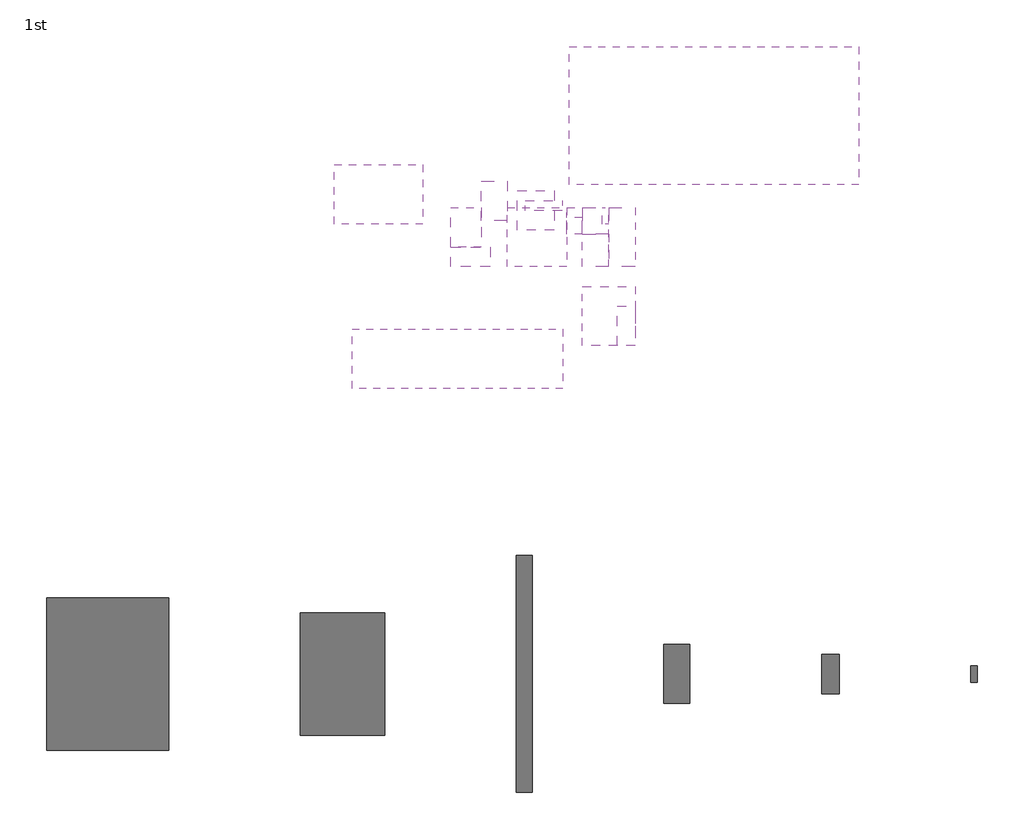
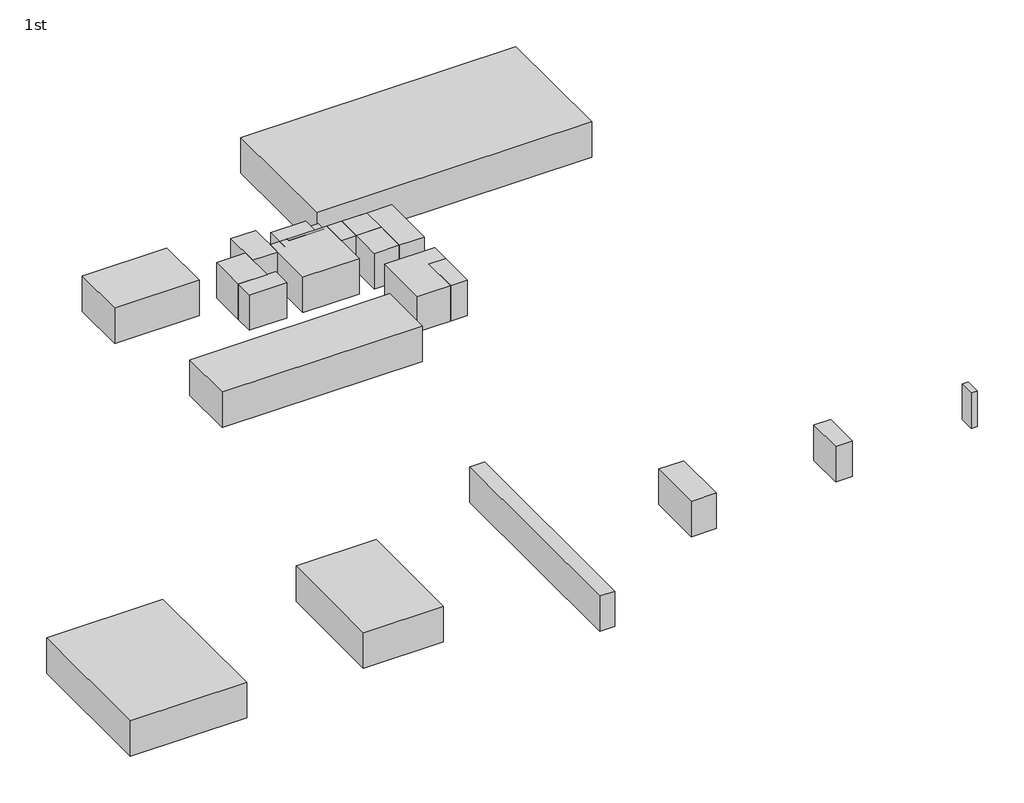
# One storey: 23 proxies.
"""IFC4 building model written with IfcOpenShell, lengths in millimetres."""

import ifcopenshell
import ifcopenshell.guid

model = None  # the IFC model being written
_history = None  # IfcOwnerHistory: only IFC2X3 demands one
_inside = {}  # id of a spatial element -> (the spatial element, [elements in it])
_under = {}  # id of a project, library or spatial element -> (it, [spatial elements below it])
_declared = {}  # id of a project -> (the project, [libraries it declares])
_typed = {}  # id of a type object -> (the type object, [elements of that type])
_made_of = {}  # id of a material, layer set ... -> (it, [elements and type objects made of it])


def new_model(schema):
    """Start an empty IFC model of exactly this schema.

    Asked for "IFC4X3", IfcOpenShell would pick the latest addendum, in which some entities
    have other attributes; the version numbers below select the first issue.
    IFC2X3 requires an IfcOwnerHistory on every rooted entity: one is made here for all.
    """
    global model, _history
    if schema == "IFC4X3":
        model = ifcopenshell.file(schema_version=(4, 3, 0, 0))
    else:
        model = ifcopenshell.file(schema=schema)
    _inside.clear()
    _under.clear()
    _declared.clear()
    _typed.clear()
    _made_of.clear()
    _history = None
    if model.schema == "IFC2X3":
        org = make("IfcOrganization", Name="unknown")
        user = make(
            "IfcPersonAndOrganization",
            ThePerson=make("IfcPerson", FamilyName="unknown"),
            TheOrganization=org,
        )
        app = make(
            "IfcApplication",
            ApplicationDeveloper=org,
            Version="unknown",
            ApplicationFullName="unknown",
            ApplicationIdentifier="unknown",
        )
        _history = make(
            "IfcOwnerHistory",
            OwningUser=user,
            OwningApplication=app,
            ChangeAction="ADDED",
            CreationDate=0,
        )
    return model


def make(cls, **values):
    """One entity of the class cls with the attributes given. An attribute that is None is left unset."""
    return model.create_entity(
        cls, **{name: value for name, value in values.items() if value is not None}
    )


def rooted(cls, **values):
    """An entity with a GlobalId (a new one), such as an element, a storey or a relation."""
    return make(cls, GlobalId=ifcopenshell.guid.new(), OwnerHistory=_history, **values)


def si_unit(unit_type, name, prefix=None):
    """IfcSIUnit, for example si_unit("LENGTHUNIT", "METRE", prefix="MILLI")."""
    return make("IfcSIUnit", UnitType=unit_type, Prefix=prefix, Name=name)


def assignment(units):
    """IfcUnitAssignment: the units of a project."""
    return None if units is None else make("IfcUnitAssignment", Units=units)


def point(xyz):
    """IfcCartesianPoint."""
    return None if xyz is None else make("IfcCartesianPoint", Coordinates=xyz)


def direction(xyz):
    """IfcDirection."""
    return None if xyz is None else make("IfcDirection", DirectionRatios=xyz)


def frame(location, z_axis=None, x_axis=None):
    """IfcAxis2Placement3D, a coordinate frame: its origin and axes. An axis left out is left unset."""
    return make(
        "IfcAxis2Placement3D",
        Location=point(location),
        Axis=direction(z_axis),
        RefDirection=direction(x_axis),
    )


def origin():
    """The frame at (0, 0, 0) with its axes left unset."""
    return frame((0.0, 0.0, 0.0))


def origin_with_axes():
    """The frame at (0, 0, 0) with the z axis (0, 0, 1) and the x axis (1, 0, 0) written out."""
    return frame((0.0, 0.0, 0.0), z_axis=(0.0, 0.0, 1.0), x_axis=(1.0, 0.0, 0.0))


def place(relative_to, where):
    """IfcLocalPlacement: puts the frame where relative to a parent placement (None: the world)."""
    return make(
        "IfcLocalPlacement", PlacementRelTo=relative_to, RelativePlacement=where
    )


def context(
    kind, dimensions, precision=None, world=None, true_north=None, identifier=None
):
    """IfcGeometricRepresentationContext, for example the 3D "Model" context."""
    return make(
        "IfcGeometricRepresentationContext",
        ContextIdentifier=identifier,
        ContextType=kind,
        CoordinateSpaceDimension=dimensions,
        Precision=precision,
        WorldCoordinateSystem=world,
        TrueNorth=true_north,
    )


def project(units=None, contexts=None):
    """IfcProject with its units and contexts."""
    return rooted(
        "IfcProject",
        Name="project",
        RepresentationContexts=contexts,
        UnitsInContext=assignment(units),
    )


def spatial(cls, under=None, at=None, **own):
    """A site, building, storey or space (cls), placed at a placement, below another one or the project."""
    s = rooted(cls, ObjectPlacement=at, **own)
    if under is not None:
        _under.setdefault(under.id(), (under, []))[1].append(s)
    return s


def polyline(points):
    """IfcPolyline through the points."""
    return make("IfcPolyline", Points=[point(p) for p in points])


def outline(outer, holes=None, kind="AREA"):
    """IfcArbitraryClosedProfileDef: a profile drawn as a closed curve; with holes, ...WithVoids."""
    if holes is None:
        return make("IfcArbitraryClosedProfileDef", ProfileType=kind, OuterCurve=outer)
    return make(
        "IfcArbitraryProfileDefWithVoids",
        ProfileType=kind,
        OuterCurve=outer,
        InnerCurves=holes,
    )


def extrude(swept, where, along, depth):
    """IfcExtrudedAreaSolid: the profile swept, set in the frame where, extruded along a direction by depth."""
    return make(
        "IfcExtrudedAreaSolid",
        SweptArea=swept,
        Position=where,
        ExtrudedDirection=direction(along),
        Depth=depth,
    )


def shape(context_of_items, identifier, shape_type, items):
    """IfcShapeRepresentation: the items that make up one representation, for example the "Body"."""
    return make(
        "IfcShapeRepresentation",
        ContextOfItems=context_of_items,
        RepresentationIdentifier=identifier,
        RepresentationType=shape_type,
        Items=items,
    )


def source(mapping_origin, context_of_items, identifier, shape_type, items):
    """IfcRepresentationMap: a shape defined once, which mapped items show again and again."""
    return make(
        "IfcRepresentationMap",
        MappingOrigin=mapping_origin,
        MappedRepresentation=shape(context_of_items, identifier, shape_type, items),
    )


def transform(
    local_origin,
    x_axis=None,
    y_axis=None,
    z_axis=None,
    scale=None,
    scale2=None,
    scale3=None,
    uniform=True,
):
    """IfcCartesianTransformationOperator3D, or its non-uniform kind. x_axis, y_axis, z_axis: its Axis1, 2, 3."""
    if uniform:
        return make(
            "IfcCartesianTransformationOperator3D",
            Axis1=direction(x_axis),
            Axis2=direction(y_axis),
            LocalOrigin=point(local_origin),
            Scale=scale,
            Axis3=direction(z_axis),
        )
    return make(
        "IfcCartesianTransformationOperator3DnonUniform",
        Axis1=direction(x_axis),
        Axis2=direction(y_axis),
        LocalOrigin=point(local_origin),
        Scale=scale,
        Axis3=direction(z_axis),
        Scale2=scale2,
        Scale3=scale3,
    )


def mapped(mapping_source, mapping_target):
    """IfcMappedItem: shows the shape of a source again, moved by a transform."""
    return make(
        "IfcMappedItem", MappingSource=mapping_source, MappingTarget=mapping_target
    )


def made_of(thing, what):
    """Note that an element or type object is made of a material, layer set ...; save() writes the relation."""
    if what is not None:
        _made_of.setdefault(what.id(), (what, []))[1].append(thing)
    return thing


def element(
    cls,
    number,
    at=None,
    inside=None,
    cuts=None,
    type_object=None,
    material=None,
    context=None,
    identifier="Body",
    shape_type=None,
    held_by="IfcProductDefinitionShape",
    body=None,
    shapes=None,
    **own,
):
    """One element of the class cls, such as IfcWall. Its Tag is "e" and its number.

    at: its placement. inside: the storey or other place that contains it. cuts: it is an
    opening in that element (IfcRelVoidsElement). A single representation is given by context,
    identifier, shape_type and body (its items); several are given by shapes. held_by: the class
    of the entity that holds the representations. save() writes the other relations.
    """
    e = rooted(cls, Tag="e%d" % number, ObjectPlacement=at, **own)
    if body is not None:
        shapes = [shape(context, identifier, shape_type, body)]
    if shapes is not None:
        e.Representation = make(held_by, Representations=shapes)
    if inside is not None:
        _inside.setdefault(inside.id(), (inside, []))[1].append(e)
    if cuts is not None:
        rooted(
            "IfcRelVoidsElement", RelatingBuildingElement=cuts, RelatedOpeningElement=e
        )
    if type_object is not None:
        _typed.setdefault(type_object.id(), (type_object, []))[1].append(e)
    return made_of(e, material)


def aggregate(whole, parts):
    """IfcRelAggregates: a whole, such as a stair, and the parts it consists of."""
    return rooted("IfcRelAggregates", RelatingObject=whole, RelatedObjects=parts)


def save(model, path):
    """Write the relations noted so far, then the file.

    IfcRelAggregates (storeys below a building ...), IfcRelContainedInSpatialStructure (elements
    in a storey), IfcRelDefinesByType, IfcRelAssociatesMaterial and IfcRelDeclares: one each for
    every whole, place, type object, material and project.
    """
    for whole, parts in _under.values():
        aggregate(whole, parts)
    for where, things in _inside.values():
        rooted(
            "IfcRelContainedInSpatialStructure",
            RelatedElements=things,
            RelatingStructure=where,
        )
    for kind, things in _typed.values():
        rooted("IfcRelDefinesByType", RelatedObjects=things, RelatingType=kind)
    for what, things in _made_of.values():
        rooted("IfcRelAssociatesMaterial", RelatedObjects=things, RelatingMaterial=what)
    for by, libraries in _declared.values():
        rooted("IfcRelDeclares", RelatingContext=by, RelatedDefinitions=libraries)
    model.write(path)


def generic_models_29bcd6f9(model_context):
    return source(origin(), model_context, "Body", "SweptSolid", [
        extrude(outline(polyline([(2000.0, 4500.0), (2000.0, -4500.0), (-2000.0, -4500.0), (-2000.0, 4500.0), (2000.0, 4500.0)])), origin_with_axes(), (0.0, 0.0, 1.0), 6000.0),
    ])


def generic_models_d82b1902(model_context):
    return source(origin(), model_context, "Body", "SweptSolid", [
        extrude(outline(polyline([(9300.0, 11600.0), (9300.0, -11600.0), (-9300.0, -11600.0), (-9300.0, 11600.0), (9300.0, 11600.0)])), origin_with_axes(), (0.0, 0.0, 1.0), 6000.0),
    ])


def generic_models_21711933(model_context):
    return source(origin(), model_context, "Body", "SweptSolid", [
        extrude(outline(polyline([(6400.0, 9300.0), (6400.0, -9300.0), (-6400.0, -9300.0), (-6400.0, 9300.0), (6400.0, 9300.0)])), origin_with_axes(), (0.0, 0.0, 1.0), 6000.0),
    ])


def generic_models_03d31222(model_context):
    return source(origin(), model_context, "Body", "SweptSolid", [
        extrude(outline(polyline([(1200.0, 18000.0), (1200.0, -18000.0), (-1200.0, -18000.0), (-1200.0, 18000.0), (1200.0, 18000.0)])), origin_with_axes(), (0.0, 0.0, 1.0), 6000.0),
    ])


def generic_models_5634f436(model_context):
    return source(origin(), model_context, "Body", "SweptSolid", [
        extrude(outline(polyline([(1350.0, 3000.0), (1350.0, -3000.0), (-1350.0, -3000.0), (-1350.0, 3000.0), (1350.0, 3000.0)])), origin_with_axes(), (0.0, 0.0, 1.0), 6000.0),
    ])


def generic_models_71e2440f(model_context):
    return source(origin(), model_context, "Body", "SweptSolid", [
        extrude(outline(polyline([(500.0, 1250.0), (500.0, -1250.0), (-500.0, -1250.0), (-500.0, 1250.0), (500.0, 1250.0)])), origin_with_axes(), (0.0, 0.0, 1.0), 6000.0),
    ])


def generic_models_57c7875f(model_context):
    return source(origin(), model_context, "Body", "SweptSolid", [
        extrude(outline(polyline([(4500.0, 16000.0), (4500.0, -16000.0), (-4500.0, -16000.0), (-4500.0, 16000.0), (4500.0, 16000.0)])), origin_with_axes(), (0.0, 0.0, 1.0), 6000.0),
    ])


def generic_models_7bff30ad(model_context):
    return source(origin(), model_context, "Body", "SweptSolid", [
        extrude(outline(polyline([(2000.0, 2000.0), (2000.0, -2000.0), (-2000.0, -2000.0), (-2000.0, 2000.0), (2000.0, 2000.0)])), origin_with_axes(), (0.0, 0.0, 1.0), 6000.0),
    ])


def generic_models_5b7b272c(model_context):
    return source(origin(), model_context, "Body", "SweptSolid", [
        extrude(outline(polyline([(2000.0, 2500.0), (2000.0, -2500.0), (-2000.0, -2500.0), (-2000.0, 2500.0), (2000.0, 2500.0)])), origin_with_axes(), (0.0, 0.0, 1.0), 6000.0),
    ])


def generic_models_47b98be1(model_context):
    return source(origin(), model_context, "Body", "SweptSolid", [
        extrude(outline(polyline([(1200.0, 2000.0), (1200.0, -2000.0), (-1200.0, -2000.0), (-1200.0, 2000.0), (1200.0, 2000.0)])), origin_with_axes(), (0.0, 0.0, 1.0), 6000.0),
    ])


def generic_models_7a053eeb(model_context):
    return source(origin(), model_context, "Body", "SweptSolid", [
        extrude(outline(polyline([(1200.0, 750.0), (1200.0, -750.0), (-1200.0, -750.0), (-1200.0, 750.0), (1200.0, 750.0)])), origin_with_axes(), (0.0, 0.0, 1.0), 6000.0),
    ])


def generic_models_ec17d728(model_context):
    return source(origin(), model_context, "Body", "SweptSolid", [
        extrude(outline(polyline([(2800.0, 3000.0), (2800.0, -3000.0), (-2800.0, -3000.0), (-2800.0, 3000.0), (2800.0, 3000.0)])), origin_with_axes(), (0.0, 0.0, 1.0), 6000.0),
    ])


def generic_models_85897e09(model_context):
    return source(origin(), model_context, "Body", "SweptSolid", [
        extrude(outline(polyline([(2800.0, 750.0), (2800.0, -750.0), (-2800.0, -750.0), (-2800.0, 750.0), (2800.0, 750.0)])), origin_with_axes(), (0.0, 0.0, 1.0), 6000.0),
    ])


def generic_models_b79df083(model_context):
    return source(origin(), model_context, "Body", "SweptSolid", [
        extrude(outline(polyline([(4500.0, 4500.0), (4500.0, -4500.0), (-4500.0, -4500.0), (-4500.0, 4500.0), (4500.0, 4500.0)])), origin_with_axes(), (0.0, 0.0, 1.0), 6000.0),
    ])


def generic_models_98b71764(model_context):
    return source(origin(), model_context, "Body", "SweptSolid", [
        extrude(outline(polyline([(2000.0, 3000.0), (2000.0, -3000.0), (-2000.0, -3000.0), (-2000.0, 3000.0), (2000.0, 3000.0)])), origin_with_axes(), (0.0, 0.0, 1.0), 6000.0),
    ])


def generic_models_1a87c0f4(model_context):
    return source(origin(), model_context, "Body", "SweptSolid", [
        extrude(outline(polyline([(2300.0, 3000.0), (2300.0, -3000.0), (-2300.0, -3000.0), (-2300.0, 3000.0), (2300.0, 3000.0)])), origin_with_axes(), (0.0, 0.0, 1.0), 6000.0),
    ])


def generic_models_df3bc381(model_context):
    return source(origin(), model_context, "Body", "SweptSolid", [
        extrude(outline(polyline([(4500.0, 6750.0), (4500.0, -6750.0), (-4500.0, -6750.0), (-4500.0, 6750.0), (4500.0, 6750.0)])), origin_with_axes(), (0.0, 0.0, 1.0), 6000.0),
    ])


def generic_models_542cc789(model_context):
    return source(origin(), model_context, "Body", "SweptSolid", [
        extrude(outline(polyline([(1500.0, 3000.0), (1500.0, -3000.0), (-1500.0, -3000.0), (-1500.0, 3000.0), (1500.0, 3000.0)])), origin_with_axes(), (0.0, 0.0, 1.0), 6000.0),
    ])


def generic_models_4d084078(model_context):
    return source(origin(), model_context, "Body", "SweptSolid", [
        extrude(outline(polyline([(4000.0, 4500.0), (4000.0, -4500.0), (-4000.0, -4500.0), (-4000.0, 4500.0), (4000.0, 4500.0)])), origin_with_axes(), (0.0, 0.0, 1.0), 6000.0),
    ])


def generic_models_7e8091d6(model_context):
    return source(origin(), model_context, "Body", "SweptSolid", [
        extrude(outline(polyline([(22000.0, 10500.0), (22000.0, -10500.0), (-22000.0, -10500.0), (-22000.0, 10500.0), (22000.0, 10500.0)])), origin_with_axes(), (0.0, 0.0, 1.0), 6000.0),
    ])


model = new_model("IFC4")

# Units and contexts
model_context = context("Model", 3, world=origin())
ifc_project = project(units=[si_unit("LENGTHUNIT", "METRE", prefix="MILLI")], contexts=[model_context])

# Site, building, storey
site = spatial("IfcSite", under=ifc_project)
building = spatial("IfcBuilding", under=site)
storey = spatial("IfcBuildingStorey", under=building, Name="1st", Elevation=6000.0)

# Proxies
placement = place(None, origin())
generic_models_shape = generic_models_29bcd6f9(model_context)
element("IfcBuildingElementProxy", 1, Name="Space Planning Box_hec : Space Planning Box_hec", ObjectType="Space Planning Box_hec : Space Planning Box_hec", at=placement, inside=storey, context=model_context, shape_type="MappedRepresentation", body=[
    mapped(generic_models_shape, transform((95800.0, 114000.0, 6000.0), x_axis=(1.0, 0.0, 0.0), y_axis=(0.0, 1.0, 0.0), z_axis=(0.0, 0.0, 1.0))),
])
element("IfcBuildingElementProxy", 2, Name="Space Planning Box_hec : Space Planning Box_hec", ObjectType="Space Planning Box_hec : Space Planning Box_hec", at=placement, inside=storey, context=model_context, shape_type="MappedRepresentation", body=[
    mapped(generic_models_shape, transform((87459.6521483, 180423.8614395, 12000.0), x_axis=(1.0, 0.0, 0.0), y_axis=(0.0, 1.0, 0.0), z_axis=(0.0, 0.0, 1.0))),
])
generic_models_2_shape = generic_models_d82b1902(model_context)
element("IfcBuildingElementProxy", 3, Name="Space Planning Box_hec : Space Planning Box_hec", ObjectType="Space Planning Box_hec : Space Planning Box_hec", at=placement, inside=storey, context=model_context, shape_type="MappedRepresentation", body=[
    mapped(generic_models_2_shape, transform((9300.0, 114000.0, 6000.0), x_axis=(1.0, 0.0, 0.0), y_axis=(0.0, 1.0, 0.0), z_axis=(0.0, 0.0, 1.0))),
])
generic_models_3_shape = generic_models_21711933(model_context)
element("IfcBuildingElementProxy", 4, Name="Space Planning Box_hec : Space Planning Box_hec", ObjectType="Space Planning Box_hec : Space Planning Box_hec", at=placement, inside=storey, context=model_context, shape_type="MappedRepresentation", body=[
    mapped(generic_models_3_shape, transform((45000.0, 114000.0, 6000.0), x_axis=(1.0, 0.0, 0.0), y_axis=(0.0, 1.0, 0.0), z_axis=(0.0, 0.0, 1.0))),
])
generic_models_4_shape = generic_models_03d31222(model_context)
element("IfcBuildingElementProxy", 5, Name="Space Planning Box_hec : Space Planning Box_hec", ObjectType="Space Planning Box_hec : Space Planning Box_hec", at=placement, inside=storey, context=model_context, shape_type="MappedRepresentation", body=[
    mapped(generic_models_4_shape, transform((72600.0, 114000.0, 6000.0), x_axis=(1.0, 0.0, 0.0), y_axis=(0.0, 1.0, 0.0), z_axis=(0.0, 0.0, 1.0))),
])
generic_models_5_shape = generic_models_5634f436(model_context)
element("IfcBuildingElementProxy", 6, Name="Space Planning Box_hec : Space Planning Box_hec", ObjectType="Space Planning Box_hec : Space Planning Box_hec", at=placement, inside=storey, context=model_context, shape_type="MappedRepresentation", body=[
    mapped(generic_models_5_shape, transform((119150.0, 114000.0, 6000.0), x_axis=(1.0, 0.0, 0.0), y_axis=(0.0, 1.0, 0.0), z_axis=(0.0, 0.0, 1.0))),
])
element("IfcBuildingElementProxy", 7, Name="Space Planning Box_hec : Space Planning Box_hec", ObjectType="Space Planning Box_hec : Space Planning Box_hec", at=placement, inside=storey, context=model_context, shape_type="MappedRepresentation", body=[
    mapped(generic_models_5_shape, transform((88109.6521483, 166923.8614395, 12000.0), x_axis=(1.0, 0.0, 0.0), y_axis=(0.0, 1.0, 0.0), z_axis=(0.0, 0.0, 1.0))),
])
generic_models_6_shape = generic_models_71e2440f(model_context)
element("IfcBuildingElementProxy", 8, Name="Space Planning Box_hec : Space Planning Box_hec", ObjectType="Space Planning Box_hec : Space Planning Box_hec", at=placement, inside=storey, context=model_context, shape_type="MappedRepresentation", body=[
    mapped(generic_models_6_shape, transform((141000.0, 114000.0, 6000.0), x_axis=(1.0, 0.0, 0.0), y_axis=(0.0, 1.0, 0.0), z_axis=(0.0, 0.0, 1.0))),
])
element("IfcBuildingElementProxy", 9, Name="Space Planning Box_hec : Space Planning Box_hec", ObjectType="Space Planning Box_hec : Space Planning Box_hec", at=placement, inside=storey, context=model_context, shape_type="MappedRepresentation", body=[
    mapped(generic_models_6_shape, transform((84959.6521483, 183673.8614395, 12000.0), x_axis=(1.0, 0.0, 0.0), y_axis=(0.0, 1.0, 0.0), z_axis=(0.0, 0.0, 1.0))),
])
generic_models_7_shape = generic_models_57c7875f(model_context)
element("IfcBuildingElementProxy", 10, Name="Space Planning Box_hec : Space Planning Box_hec", ObjectType="Space Planning Box_hec : Space Planning Box_hec", at=placement, inside=storey, context=model_context, shape_type="MappedRepresentation", body=[
    mapped(generic_models_7_shape, transform((62459.6521483, 161923.8614395, 12000.0), x_axis=(0.0, -1.0, 0.0), y_axis=(1.0, 0.0, 0.0), z_axis=(0.0, 0.0, 1.0))),
])
generic_models_8_shape = generic_models_7bff30ad(model_context)
element("IfcBuildingElementProxy", 11, Name="Space Planning Box_hec : Space Planning Box_hec", ObjectType="Space Planning Box_hec : Space Planning Box_hec", at=placement, inside=storey, context=model_context, shape_type="MappedRepresentation", body=[
    mapped(generic_models_8_shape, transform((83459.6521483, 182923.8614395, 12000.0), x_axis=(1.0, 0.0, 0.0), y_axis=(0.0, 1.0, 0.0), z_axis=(0.0, 0.0, 1.0))),
])
generic_models_9_shape = generic_models_5b7b272c(model_context)
element("IfcBuildingElementProxy", 12, Name="Space Planning Box_hec : Space Planning Box_hec", ObjectType="Space Planning Box_hec : Space Planning Box_hec", at=placement, inside=storey, context=model_context, shape_type="MappedRepresentation", body=[
    mapped(generic_models_9_shape, transform((83459.6521483, 178423.8614395, 12000.0), x_axis=(1.0, 0.0, 0.0), y_axis=(0.0, 1.0, 0.0), z_axis=(0.0, 0.0, 1.0))),
])
generic_models_10_shape = generic_models_47b98be1(model_context)
element("IfcBuildingElementProxy", 13, Name="Space Planning Box_hec : Space Planning Box_hec", ObjectType="Space Planning Box_hec : Space Planning Box_hec", at=placement, inside=storey, context=model_context, shape_type="MappedRepresentation", body=[
    mapped(generic_models_10_shape, transform((80259.6521483, 182923.8614395, 12000.0), x_axis=(1.0, 0.0, 0.0), y_axis=(0.0, 1.0, 0.0), z_axis=(0.0, 0.0, 1.0))),
])
generic_models_11_shape = generic_models_7a053eeb(model_context)
element("IfcBuildingElementProxy", 14, Name="Space Planning Box_hec : Space Planning Box_hec", ObjectType="Space Planning Box_hec : Space Planning Box_hec", at=placement, inside=storey, context=model_context, shape_type="MappedRepresentation", body=[
    mapped(generic_models_11_shape, transform((80259.6521483, 184173.8614395, 12000.0), x_axis=(1.0, 0.0, 0.0), y_axis=(0.0, 1.0, 0.0), z_axis=(0.0, 0.0, 1.0))),
])
generic_models_12_shape = generic_models_ec17d728(model_context)
element("IfcBuildingElementProxy", 15, Name="Space Planning Box_hec : Space Planning Box_hec", ObjectType="Space Planning Box_hec : Space Planning Box_hec", at=placement, inside=storey, context=model_context, shape_type="MappedRepresentation", body=[
    mapped(generic_models_12_shape, transform((74362.3489007, 184480.7589148, 12000.0), x_axis=(1.0, 0.0, 0.0), y_axis=(0.0, 1.0, 0.0), z_axis=(0.0, 0.0, 1.0))),
])
generic_models_13_shape = generic_models_85897e09(model_context)
element("IfcBuildingElementProxy", 16, Name="Space Planning Box_hec : Space Planning Box_hec", ObjectType="Space Planning Box_hec : Space Planning Box_hec", at=placement, inside=storey, context=model_context, shape_type="MappedRepresentation", body=[
    mapped(generic_models_13_shape, transform((75555.0538314, 185230.7589148, 12000.0), x_axis=(1.0, 0.0, 0.0), y_axis=(0.0, 1.0, 0.0), z_axis=(0.0, 0.0, 1.0))),
])
generic_models_14_shape = generic_models_b79df083(model_context)
element("IfcBuildingElementProxy", 17, Name="Space Planning Box_hec : Space Planning Box_hec", ObjectType="Space Planning Box_hec : Space Planning Box_hec", at=placement, inside=storey, context=model_context, shape_type="MappedRepresentation", body=[
    mapped(generic_models_14_shape, transform((74559.6521483, 180423.8614395, 12000.0), x_axis=(1.0, 0.0, 0.0), y_axis=(0.0, 1.0, 0.0), z_axis=(0.0, 0.0, 1.0))),
])
generic_models_15_shape = generic_models_98b71764(model_context)
element("IfcBuildingElementProxy", 18, Name="Space Planning Box_hec : Space Planning Box_hec", ObjectType="Space Planning Box_hec : Space Planning Box_hec", at=placement, inside=storey, context=model_context, shape_type="MappedRepresentation", body=[
    mapped(generic_models_15_shape, transform((68059.6521483, 185923.8614395, 12000.0), x_axis=(1.0, 0.0, 0.0), y_axis=(0.0, 1.0, 0.0), z_axis=(0.0, 0.0, 1.0))),
])
generic_models_16_shape = generic_models_1a87c0f4(model_context)
element("IfcBuildingElementProxy", 19, Name="Space Planning Box_hec : Space Planning Box_hec", ObjectType="Space Planning Box_hec : Space Planning Box_hec", at=placement, inside=storey, context=model_context, shape_type="MappedRepresentation", body=[
    mapped(generic_models_16_shape, transform((63759.6521483, 181923.8614395, 12000.0), x_axis=(1.0, 0.0, 0.0), y_axis=(0.0, 1.0, 0.0), z_axis=(0.0, 0.0, 1.0))),
])
generic_models_17_shape = generic_models_df3bc381(model_context)
element("IfcBuildingElementProxy", 20, Name="Space Planning Box_hec : Space Planning Box_hec", ObjectType="Space Planning Box_hec : Space Planning Box_hec", at=placement, inside=storey, context=model_context, shape_type="MappedRepresentation", body=[
    mapped(generic_models_17_shape, transform((50459.6521483, 186923.8614395, 12000.0), x_axis=(0.0, -1.0, 0.0), y_axis=(1.0, 0.0, 0.0), z_axis=(0.0, 0.0, 1.0))),
])
generic_models_18_shape = generic_models_542cc789(model_context)
element("IfcBuildingElementProxy", 21, Name="Space Planning Box_hec : Space Planning Box_hec", ObjectType="Space Planning Box_hec : Space Planning Box_hec", at=placement, inside=storey, context=model_context, shape_type="MappedRepresentation", body=[
    mapped(generic_models_18_shape, transform((64459.6521483, 177423.8614395, 12000.0), x_axis=(0.0, -1.0, 0.0), y_axis=(1.0, 0.0, 0.0), z_axis=(0.0, 0.0, 1.0))),
])
generic_models_19_shape = generic_models_4d084078(model_context)
element("IfcBuildingElementProxy", 22, Name="Space Planning Box_hec : Space Planning Box_hec", ObjectType="Space Planning Box_hec : Space Planning Box_hec", at=placement, inside=storey, context=model_context, shape_type="MappedRepresentation", body=[
    mapped(generic_models_19_shape, transform((85459.6521483, 168423.8614395, 12000.0), x_axis=(1.0, 0.0, 0.0), y_axis=(0.0, 1.0, 0.0), z_axis=(0.0, 0.0, 1.0))),
])
generic_models_20_shape = generic_models_7e8091d6(model_context)
element("IfcBuildingElementProxy", 23, Name="Space Planning Box_hec : Space Planning Box_hec", ObjectType="Space Planning Box_hec : Space Planning Box_hec", at=placement, inside=storey, context=model_context, shape_type="MappedRepresentation", body=[
    mapped(generic_models_20_shape, transform((101459.6521483, 198923.8614395, 12000.0), x_axis=(1.0, 0.0, 0.0), y_axis=(0.0, 1.0, 0.0), z_axis=(0.0, 0.0, 1.0))),
])

save(model, "model.ifc")

# Revit data of these elements
# Type "Space Planning Box_hec : Space Planning Box_hec"
#   Type Comments = "..."
#   Room Name [instance default] = "?"
#   Interior Finish [instance default] = ""
#   Exterior Finish [instance default] = ""
#   Department [instance default] = ""
#   Assembly Code = "..."
#   Width [instance default] = 1524 mm
#   Program Area [instance default] = 0.00 m²
#   Length [instance default] = 1524 mm
#   Height [instance default] = 1524 mm
#   Area [instance default] = 2.32258 m²
#   Fill Color [instance default] = Cyan
#   Default Elevation = 0
# Element 1 (IfcBuildingElementProxy, "Space Planning Box_hec : Space Planning Box_hec")
#   Room Name = "Stairway"
#   Interior Finish = "IF2"
#   Exterior Finish = "EF1"
#   Department = "AR"
#   Width = 4000 mm
#   Program Area = 36.00 m²
#   Length = 9000 mm
#   Height = 6000 mm
#   Area = 36.00 m²
#   Fill Color = Lavender
#   Phase Created = New Construction
#   Materials on its faces: "Lavender"
# Element 2 (IfcBuildingElementProxy, "Space Planning Box_hec : Space Planning Box_hec")
#   Room Name = "Stairway"
#   Interior Finish = "IF2"
#   Exterior Finish = "EF1"
#   Department = "AR"
#   Width = 4000 mm
#   Program Area = 38.00 m²
#   Length = 9000 mm
#   Height = 6000 mm
#   Area = 36.00 m²
#   Fill Color = Lavender
#   Phase Created = New Construction
#   Materials on its faces: "Lavender"
# Element 3 (IfcBuildingElementProxy, "Space Planning Box_hec : Space Planning Box_hec")
#   Room Name = "Electronic Room"
#   Interior Finish = "IF1"
#   Exterior Finish = "EF1"
#   Department = "CI"
#   Width = 18600 mm
#   Program Area = 431.52 m²
#   Length = 23200 mm
#   Height = 6000 mm
#   Area = 431.52 m²
#   Fill Color = Lime
#   Phase Created = New Construction
#   Materials on its faces: "Lime"
# Element 4 (IfcBuildingElementProxy, "Space Planning Box_hec : Space Planning Box_hec")
#   Room Name = "Electrical Room"
#   Interior Finish = "IF1"
#   Exterior Finish = "EF1"
#   Department = "EL"
#   Width = 12800 mm
#   Program Area = 238.08 m²
#   Length = 18600 mm
#   Height = 6000 mm
#   Area = 238.08 m²
#   Fill Color = Blue
#   Phase Created = New Construction
#   Materials on its faces: "Blue"
# Element 5 (IfcBuildingElementProxy, "Space Planning Box_hec : Space Planning Box_hec")
#   Room Name = "Corridor"
#   Interior Finish = "IF2-1"
#   Exterior Finish = "EF1"
#   Department = "AR"
#   Width = 2400 mm
#   Program Area = 86.40 m²
#   Length = 36000 mm
#   Height = 6000 mm
#   Area = 86.40 m²
#   Fill Color = Lavender
#   Phase Created = New Construction
#   Materials on its faces: "Lavender"
# Elements 6, 7 (IfcBuildingElementProxy, "Space Planning Box_hec : Space Planning Box_hec")
#   Room Name = "Duct Shaft"
#   Interior Finish = "NA"
#   Exterior Finish = "EF1"
#   Department = "HV"
#   Width = 2700 mm
#   Program Area = 16.20 m²
#   Length = 6000 mm
#   Height = 6000 mm
#   Area = 16.20 m²
#   Fill Color = Pink
#   Phase Created = New Construction
#   Materials on its faces: "Pink"
# Elements 8, 9 (IfcBuildingElementProxy, "Space Planning Box_hec : Space Planning Box_hec")
#   Room Name = "Pipe Shaft"
#   Interior Finish = "NA"
#   Exterior Finish = "EF1"
#   Department = "HV"
#   Width = 1000 mm
#   Program Area = 2.50 m²
#   Length = 2500 mm
#   Height = 6000 mm
#   Area = 2.50 m²
#   Fill Color = Pink
#   Phase Created = New Construction
#   Materials on its faces: "Pink"
# Element 10 (IfcBuildingElementProxy, "Space Planning Box_hec : Space Planning Box_hec")
#   Room Name = "Central Control Room"
#   Interior Finish = "IF3"
#   Exterior Finish = "EF1"
#   Department = "CI"
#   Width = 9000 mm
#   Program Area = 288.00 m²
#   Length = 32000 mm
#   Height = 6000 mm
#   Area = 288.00 m²
#   Fill Color = Lime
#   Phase Created = New Construction
#   Materials on its faces: "Lime"
# Element 11 (IfcBuildingElementProxy, "Space Planning Box_hec : Space Planning Box_hec")
#   Room Name = "Toilet (F)"
#   Interior Finish = "IF5"
#   Exterior Finish = "EF1"
#   Department = "AR"
#   Width = 4000 mm
#   Program Area = 72.00 m²
#   Length = 4000 mm
#   Height = 6000 mm
#   Area = 16.00 m²
#   Fill Color = Lavender
#   Phase Created = New Construction
#   Materials on its faces: "Lavender"
# Element 12 (IfcBuildingElementProxy, "Space Planning Box_hec : Space Planning Box_hec")
#   Room Name = "Toilet (M)"
#   Interior Finish = "IF5"
#   Exterior Finish = "EF1"
#   Department = "AR"
#   Width = 4000 mm
#   Program Area = 72.00 m²
#   Length = 5000 mm
#   Height = 6000 mm
#   Area = 20.00 m²
#   Fill Color = Lavender
#   Phase Created = New Construction
#   Materials on its faces: "Lavender"
# Element 13 (IfcBuildingElementProxy, "Space Planning Box_hec : Space Planning Box_hec")
#   Room Name = "Locker Room (F)"
#   Interior Finish = "IF2-1"
#   Exterior Finish = "EF1"
#   Department = "AR"
#   Width = 2400 mm
#   Program Area = 31.50 m²
#   Length = 4000 mm
#   Height = 6000 mm
#   Area = 9.60 m²
#   Fill Color = Lavender
#   Phase Created = New Construction
#   Materials on its faces: "Lavender"
# Element 14 (IfcBuildingElementProxy, "Space Planning Box_hec : Space Planning Box_hec")
#   Room Name = "Shower Room (F)"
#   Interior Finish = "IF5"
#   Exterior Finish = "EF1"
#   Department = "AR"
#   Width = 2400 mm
#   Program Area = 31.50 m²
#   Length = 1500 mm
#   Height = 6000 mm
#   Area = 3.60 m²
#   Fill Color = Lavender
#   Phase Created = New Construction
#   Materials on its faces: "Lavender"
# Element 15 (IfcBuildingElementProxy, "Space Planning Box_hec : Space Planning Box_hec")
#   Room Name = "Locker Room (M)"
#   Interior Finish = "IF2-1"
#   Exterior Finish = "EF1"
#   Department = "AR"
#   Width = 5600 mm
#   Program Area = 31.50 m²
#   Length = 6000 mm
#   Height = 6000 mm
#   Area = 33.60 m²
#   Fill Color = Lavender
#   Phase Created = New Construction
#   Materials on its faces: "Lavender"
# Element 16 (IfcBuildingElementProxy, "Space Planning Box_hec : Space Planning Box_hec")
#   Room Name = "Shower Room (M)"
#   Interior Finish = "IF5"
#   Exterior Finish = "EF1"
#   Department = "AR"
#   Width = 5600 mm
#   Program Area = 31.50 m²
#   Length = 1500 mm
#   Height = 6000 mm
#   Area = 8.40 m²
#   Fill Color = Lavender
#   Phase Created = New Construction
#   Materials on its faces: "Lavender"
# Element 17 (IfcBuildingElementProxy, "Space Planning Box_hec : Space Planning Box_hec")
#   Room Name = "Kitch & Lunch Room"
#   Interior Finish = "IF2-1"
#   Exterior Finish = "EF1"
#   Department = "AR"
#   Width = 9000 mm
#   Program Area = 31.50 m²
#   Length = 9000 mm
#   Height = 6000 mm
#   Area = 81.00 m²
#   Fill Color = Lavender
#   Phase Created = New Construction
#   Materials on its faces: "Lavender"
# Element 18 (IfcBuildingElementProxy, "Space Planning Box_hec : Space Planning Box_hec")
#   Room Name = "Shift Office Room"
#   Interior Finish = "IF2-1"
#   Exterior Finish = "EF1"
#   Department = "AR"
#   Width = 4000 mm
#   Program Area = 43.20 m²
#   Length = 6000 mm
#   Height = 6000 mm
#   Area = 24.00 m²
#   Fill Color = Lavender
#   Phase Created = New Construction
#   Materials on its faces: "Lavender"
# Element 19 (IfcBuildingElementProxy, "Space Planning Box_hec : Space Planning Box_hec")
#   Room Name = "Document Room"
#   Interior Finish = "IF2-1"
#   Exterior Finish = "EF1"
#   Department = "AR"
#   Width = 4600 mm
#   Program Area = 48.00 m²
#   Length = 6000 mm
#   Height = 6000 mm
#   Area = 27.60 m²
#   Fill Color = Lavender
#   Phase Created = New Construction
#   Materials on its faces: "Lavender"
# Element 20 (IfcBuildingElementProxy, "Space Planning Box_hec : Space Planning Box_hec")
#   Room Name = "Engineer Room"
#   Interior Finish = "IF3"
#   Exterior Finish = "EF1"
#   Department = "CI"
#   Width = 9000 mm
#   Program Area = 120.00 m²
#   Length = 13500 mm
#   Height = 6000 mm
#   Area = 121.50 m²
#   Fill Color = Lime
#   Phase Created = New Construction
#   Materials on its faces: "Lime"
# Element 21 (IfcBuildingElementProxy, "Space Planning Box_hec : Space Planning Box_hec")
#   Room Name = "LOTO Office Room"
#   Interior Finish = "IF2-1"
#   Exterior Finish = "EF1"
#   Department = "AR"
#   Width = 3000 mm
#   Program Area = 31.50 m²
#   Length = 6000 mm
#   Height = 6000 mm
#   Area = 18.00 m²
#   Fill Color = Lavender
#   Phase Created = New Construction
#   Materials on its faces: "Lavender"
# Element 22 (IfcBuildingElementProxy, "Space Planning Box_hec : Space Planning Box_hec")
#   Room Name = "Fire Gas Room"
#   Interior Finish = "IF1"
#   Exterior Finish = "EF1"
#   Department = "SF"
#   Width = 8000 mm
#   Program Area = 0.00 m²
#   Length = 9000 mm
#   Height = 6000 mm
#   Area = 72.00 m²
#   Fill Color = Cyan
#   Phase Created = New Construction
#   Materials on its faces: "Cyan"
# Element 23 (IfcBuildingElementProxy, "Space Planning Box_hec : Space Planning Box_hec")
#   Room Name = "Corridor"
#   Interior Finish = "IF2-1"
#   Exterior Finish = "EF1"
#   Department = "AR"
#   Width = 44000 mm
#   Program Area = 0.00 m²
#   Length = 21000 mm
#   Height = 6000 mm
#   Area = 924.00 m²
#   Fill Color = Lavender
#   Phase Created = New Construction
#   Materials on its faces: "Lavender"
# Materials
#   "Cyan": class "Generic", colour RGB 0 255 255, transparency 0.2, Cost = 0
#   "Lavender": class "Generic", colour RGB 186 85 211, transparency 0.2, Cost = 0
#   "Lime": class "Generic", colour RGB 0 255 0, transparency 0.2, Cost = 0
#   "Blue": class "Generic", colour RGB 0 0 255, transparency 0.2, Cost = 0
#   "Pink": class "Generic", colour RGB 255 105 180, transparency 0.2, Cost = 0
# Room at (65459.652, 168423.861) mm, phase "New Construction", upper offset 2438.4 mm, lower offset 0 mm
#   Number = "3.0"
#   Name = "a"
# Room at (54709.652, 180423.861) mm, phase "New Construction", upper offset 2438.4 mm, lower offset 0 mm
#   Number = "3.1"
#   Name = "a"
# Room at (63759.652, 181923.861) mm, phase "New Construction", upper offset 2438.4 mm, lower offset 0 mm
#   Number = "3.2"
#   Name = "a"
# Room at (83459.652, 178423.861) mm, phase "New Construction", upper offset 2438.4 mm, lower offset 0 mm
#   Number = "3.3"
#   Name = "a"
# Room at (87459.652, 180423.861) mm, phase "New Construction", upper offset 2438.4 mm, lower offset 0 mm
#   Number = "3.4"
#   Name = "a"
# Room at (68059.652, 181923.861) mm, phase "New Construction", upper offset 2438.4 mm, lower offset 0 mm
#   Number = "3.5"
#   Name = "a"
# Room at (64459.652, 177423.861) mm, phase "New Construction", upper offset 2438.4 mm, lower offset 0 mm
#   Number = "3.6"
#   Name = "a"
# Room at (80259.652, 184173.861) mm, phase "New Construction", upper offset 2438.4 mm, lower offset 0 mm
#   Number = "3.7"
#   Name = "a"
# Room at (67459.652, 174423.861) mm, phase "New Construction", upper offset 2438.4 mm, lower offset 0 mm
#   Number = "3.8"
#   Name = "a"
# Room at (80259.652, 182173.861) mm, phase "New Construction", upper offset 2438.4 mm, lower offset 0 mm
#   Number = "3.9"
#   Name = "a"
# Room at (76259.652, 184173.861) mm, phase "New Construction", upper offset 2438.4 mm, lower offset 0 mm
#   Number = "3.10"
#   Name = "a"
# Room at (74559.652, 178751.292) mm, phase "New Construction", upper offset 2438.4 mm, lower offset 0 mm
#   Number = "3.11"
#   Name = "a"
# Room at (76259.652, 181173.861) mm, phase "New Construction", upper offset 2438.4 mm, lower offset 0 mm
#   Number = "3.12"
#   Name = "a"
# Room at (85459.652, 168423.861) mm, phase "New Construction", upper offset 2438.4 mm, lower offset 0 mm
#   Number = "3.13"
#   Name = "a"
# Room at (88109.652, 166923.861) mm, phase "New Construction", upper offset 2438.4 mm, lower offset 0 mm
#   Number = "3.14"
#   Name = "a"
# Room at (83459.652, 182923.861) mm, phase "New Construction", upper offset 2438.4 mm, lower offset 0 mm
#   Number = "3.15"
#   Name = "a"
# Room at (84959.652, 183673.861) mm, phase "New Construction", upper offset 2438.4 mm, lower offset 0 mm
#   Number = "3.16"
#   Name = "a"
